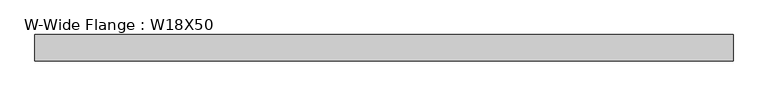
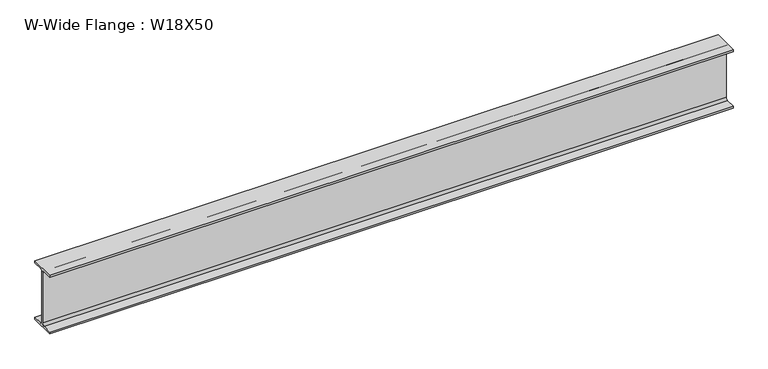
"""IFC4 building model written with IfcOpenShell, lengths in millimetres: beam geometry, W-Wide Flange : W18X50."""

from ifc_helpers import new_model, si_unit, point, frame, frame_2d, origin, place, context, project, spatial, polyline, circle_curve, trimmed, segment, composite_curve, outline, extrude, source, transform, mapped, element, save


def w_wide_flange_w18x50_3a8a2cf8(model_context):
    return source(origin(), model_context, "Body", "SweptSolid", [
        extrude(outline(composite_curve([segment(polyline([(95.25, -214.122), (95.25, -228.6), (-95.25, -228.6), (-95.25, -214.122), (-21.7805, -214.122)]), True, "CONTINUOUS"), segment(trimmed(circle_curve(frame_2d((-21.7805, -196.85)), 17.272), [point((-21.7805, -214.122))], [point((-4.5085, -196.85))], True, "CARTESIAN"), True, "CONTINUOUS"), segment(polyline([(-4.5085, -196.85), (-4.5085, 196.85)]), True, "CONTINUOUS"), segment(trimmed(circle_curve(frame_2d((-21.7805, 196.85)), 17.272), [point((-4.5085, 196.85))], [point((-21.7805, 214.122))], True, "CARTESIAN"), True, "CONTINUOUS"), segment(polyline([(-21.7805, 214.122), (-95.25, 214.122), (-95.25, 228.6), (95.25, 228.6), (95.25, 214.122), (21.7805, 214.122)]), True, "CONTINUOUS"), segment(trimmed(circle_curve(frame_2d((21.7805, 196.85)), 17.272), [point((21.7805, 214.122))], [point((4.5085, 196.85))], True, "CARTESIAN"), True, "CONTINUOUS"), segment(polyline([(4.5085, 196.85), (4.5085, -196.85)]), True, "CONTINUOUS"), segment(trimmed(circle_curve(frame_2d((21.7805, -196.85)), 17.272), [point((4.5085, -196.85))], [point((21.7805, -214.122))], True, "CARTESIAN"), True, "CONTINUOUS"), segment(polyline([(21.7805, -214.122), (95.25, -214.122)]), True, "CONTINUOUS")], self_intersect=False)), frame((-2540.381, 0.0, 0.0), z_axis=(1.0, 0.0, 0.0), x_axis=(0.0, 1.0, 0.0)), (0.0, 0.0, 1.0), 5054.981),
    ])


if __name__ == "__main__":
    model = new_model("IFC4")
    model_context = context("Model", 3, world=origin())
    ifc_project = project(units=[si_unit("LENGTHUNIT", "METRE", prefix="MILLI")], contexts=[model_context])
    site = spatial("IfcSite", under=ifc_project)
    building = spatial("IfcBuilding", under=site)
    placement = place(None, origin())
    w_wide_flange_w18x50_shape = w_wide_flange_w18x50_3a8a2cf8(model_context)
    element("IfcBeam", 1, ObjectType="W-Wide Flange : W18X50", at=placement, inside=building, context=model_context, shape_type="MappedRepresentation", body=[
        mapped(w_wide_flange_w18x50_shape, transform((0.0, 0.0, 0.0), x_axis=(1.0, 0.0, 0.0), y_axis=(0.0, 1.0, 0.0), z_axis=(0.0, 0.0, 1.0))),
    ])
    save(model, "model.ifc")

# Revit data of these elements
# Type "W-Wide Flange : W18X50"
#   Assembly Code = "B10"
#   W = 50
#   Length [instance default] = 5' - 0"
#   bf = 0' - 7 1/2"
#   d = 1' - 6"
#   k = 0' - 1 1/4"
#   k2 = 0' - 0.68"
#   tf = 0' - 0.57"
#   tw = 0' - 0.355"
#   A = 0.102083 SF
#   Structural Material [instance default] = Steel ASTM A992
# Element 1 (IfcBeam, "W-Wide Flange : W18X50")
#   Materials on its faces: "Steel ASTM A992"
# Materials
#   "Steel ASTM A992": class "Metal", colour RGB 199 199 199, transparency 0, Description = "Structural steel 50ksi", Cost = 0
